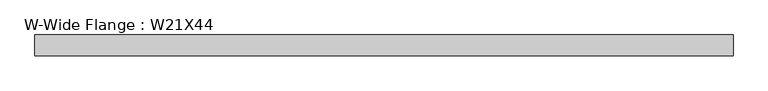
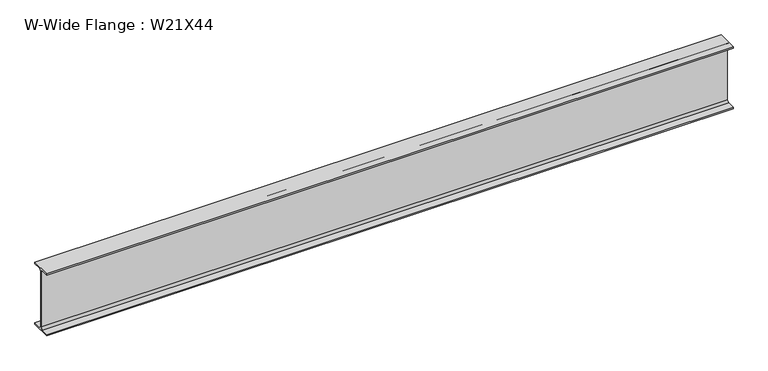
"""IFC4 building model written with IfcOpenShell, lengths in millimetres: beam geometry, W-Wide Flange : W21X44."""

from ifc_helpers import new_model, si_unit, point, frame, frame_2d, origin, place, context, project, spatial, polyline, circle_curve, trimmed, segment, composite_curve, outline, extrude, source, transform, mapped, element, save


def w_wide_flange_w21x44_175405ae(model_context):
    return source(origin(), model_context, "Body", "SweptSolid", [
        extrude(outline(composite_curve([segment(polyline([(82.55, -251.46), (82.55, -262.89), (-82.55, -262.89), (-82.55, -251.46), (-21.59, -251.46)]), True, "CONTINUOUS"), segment(trimmed(circle_curve(frame_2d((-21.59, -234.315)), 17.145), [point((-21.59, -251.46))], [point((-4.445, -234.315))], True, "CARTESIAN"), True, "CONTINUOUS"), segment(polyline([(-4.445, -234.315), (-4.445, 234.315)]), True, "CONTINUOUS"), segment(trimmed(circle_curve(frame_2d((-21.59, 234.315)), 17.145), [point((-4.445, 234.315))], [point((-21.59, 251.46))], True, "CARTESIAN"), True, "CONTINUOUS"), segment(polyline([(-21.59, 251.46), (-82.55, 251.46), (-82.55, 262.89), (82.55, 262.89), (82.55, 251.46), (21.59, 251.46)]), True, "CONTINUOUS"), segment(trimmed(circle_curve(frame_2d((21.59, 234.315)), 17.145), [point((21.59, 251.46))], [point((4.445, 234.315))], True, "CARTESIAN"), True, "CONTINUOUS"), segment(polyline([(4.445, 234.315), (4.445, -234.315)]), True, "CONTINUOUS"), segment(trimmed(circle_curve(frame_2d((21.59, -234.315)), 17.145), [point((4.445, -234.315))], [point((21.59, -251.46))], True, "CARTESIAN"), True, "CONTINUOUS"), segment(polyline([(21.59, -251.46), (82.55, -251.46)]), True, "CONTINUOUS")], self_intersect=False)), frame((-2763.8375, 0.0, 0.0), z_axis=(1.0, 0.0, 0.0), x_axis=(0.0, 1.0, 0.0)), (0.0, 0.0, 1.0), 5508.5753906),
    ])


if __name__ == "__main__":
    model = new_model("IFC4")
    model_context = context("Model", 3, world=origin())
    ifc_project = project(units=[si_unit("LENGTHUNIT", "METRE", prefix="MILLI")], contexts=[model_context])
    site = spatial("IfcSite", under=ifc_project)
    building = spatial("IfcBuilding", under=site)
    placement = place(None, origin())
    w_wide_flange_w21x44_shape = w_wide_flange_w21x44_175405ae(model_context)
    element("IfcBeam", 1, ObjectType="W-Wide Flange : W21X44", at=placement, inside=building, context=model_context, shape_type="MappedRepresentation", body=[
        mapped(w_wide_flange_w21x44_shape, transform((0.0, 0.0, 0.0), x_axis=(1.0, 0.0, 0.0), y_axis=(0.0, 1.0, 0.0), z_axis=(0.0, 0.0, 1.0))),
    ])
    save(model, "model.ifc")

# Revit data of these elements
# Type "W-Wide Flange : W21X44"
#   Assembly Code = "B10"
#   W = 44
#   Length [instance default] = 1524 mm
#   bf = 165.1 mm
#   d = 525.78 mm
#   k = 28.575 mm
#   k2 = 17.145 mm
#   tf = 11.43 mm
#   tw = 8.89 mm
#   A = 0.00838708 m²
#   Structural Material [instance default] = Steel ASTM A992
# Element 1 (IfcBeam, "W-Wide Flange : W21X44")
#   Structural Material = Aluminum, Anodized Red
#   Materials on its faces: "Aluminum, Anodized Red"
# Materials
#   "Steel ASTM A992": class "Metal", colour RGB 128 0 0, transparency 0, Description = "Structural steel 50ksi", Cost = 0
#   "Aluminum, Anodized Red": class "Metal", colour RGB 120 120 120, transparency 0, Description = "Anodized aluminum, red", Cost = 0
